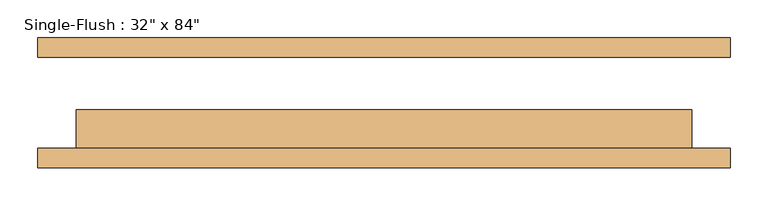
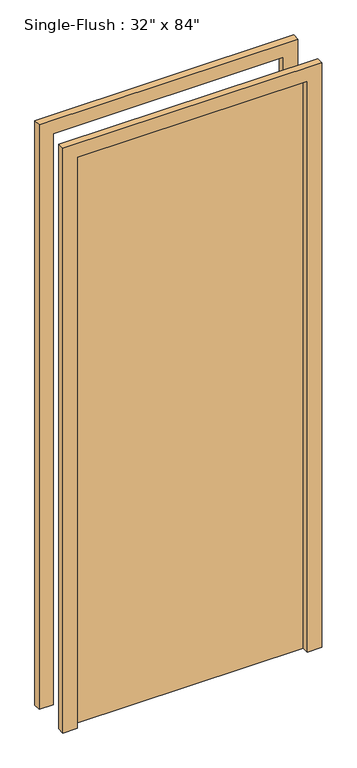
"""IFC4 building model written with IfcOpenShell, lengths in millimetres: door geometry."""

from ifc_helpers import new_model, si_unit, frame, origin, origin_with_axes, place, context, project, spatial, polyline, outline, extrude, source, transform, mapped, element, save


def door_bcb4a79f(model_context):
    return source(origin(), model_context, "Body", "SweptSolid", [
        extrude(outline(polyline([(2184.4, -457.2), (0.0, -457.2), (0.0, -406.4), (2133.6, -406.4), (2133.6, 406.4), (0.0, 406.4), (0.0, 457.2), (2184.4, 457.2), (2184.4, -457.2)])), frame((0.0, -85.725, 0.0), z_axis=(0.0, 1.0, 0.0), x_axis=(0.0, 0.0, 1.0)), (0.0, 0.0, 1.0), 25.4),
        extrude(outline(polyline([(2184.4, 457.2), (2184.4, -457.2), (0.0, -457.2), (0.0, -406.4), (2133.6, -406.4), (2133.6, 406.4), (0.0, 406.4), (0.0, 457.2), (2184.4, 457.2)])), frame((0.0, 60.325, 0.0), z_axis=(0.0, 1.0, 0.0), x_axis=(0.0, 0.0, 1.0)), (0.0, 0.0, 1.0), 25.4),
        extrude(outline(polyline([(406.4, -9.525), (406.4, -60.325), (-406.4, -60.325), (-406.4, -9.525), (406.4, -9.525)])), origin_with_axes(), (0.0, 0.0, 1.0), 2133.6),
    ])


if __name__ == "__main__":
    model = new_model("IFC4")
    model_context = context("Model", 3, world=origin())
    ifc_project = project(units=[si_unit("LENGTHUNIT", "METRE", prefix="MILLI")], contexts=[model_context])
    site = spatial("IfcSite", under=ifc_project)
    building = spatial("IfcBuilding", under=site)
    placement = place(None, origin())
    door_shape = door_bcb4a79f(model_context)
    element("IfcDoor", 1, ObjectType="Single-Flush : 32\" x 84\"", at=placement, inside=building, context=model_context, shape_type="MappedRepresentation", body=[
        mapped(door_shape, transform((0.0, 0.0, 0.0), x_axis=(1.0, 0.0, 0.0), y_axis=(0.0, 1.0, 0.0), z_axis=(0.0, 0.0, 1.0))),
    ])
    save(model, "model.ifc")

# Revit data of these elements
# Type "Single-Flush : 32\" x 84\""
#   Type Mark = "10"
#   Construction Type Id = "MDOOR"
#   Assembly Code = "C1020"
#   Analytic Construction = "Metal"
#   Thickness = 0' - 2"
#   Heat Transfer Coefficient (U) = 3.7021 W/(m²·K)
#   Height = 7' - 0"
#   Trim Projection Ext = 0' - 1"
#   Trim Projection Int = 0' - 1"
#   Trim Width = 0' - 2"
#   Width = 2' - 8"
#   Door Material = Door - Panel
#   Frame Material = Door - Frame
#   Visual Light Transmittance = 0
#   Solar Heat Gain Coefficient = 0
#   Function = (empty or 0)
#   Wall Closure = (empty or 0)
# Element 1 (IfcDoor, "Single-Flush : 32\" x 84\"")
#   Materials on its faces: "Door - Frame", "Door - Panel"
# Materials
#   "Door - Panel": class "Wood", colour RGB 212 179 113, transparency 0, Cost = 0
#   "Door - Frame": class "Miscellaneous", colour RGB 65 65 65, transparency 0, Cost = 0
